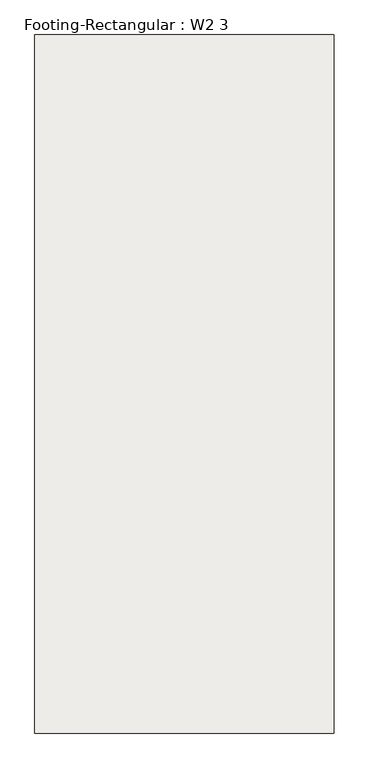
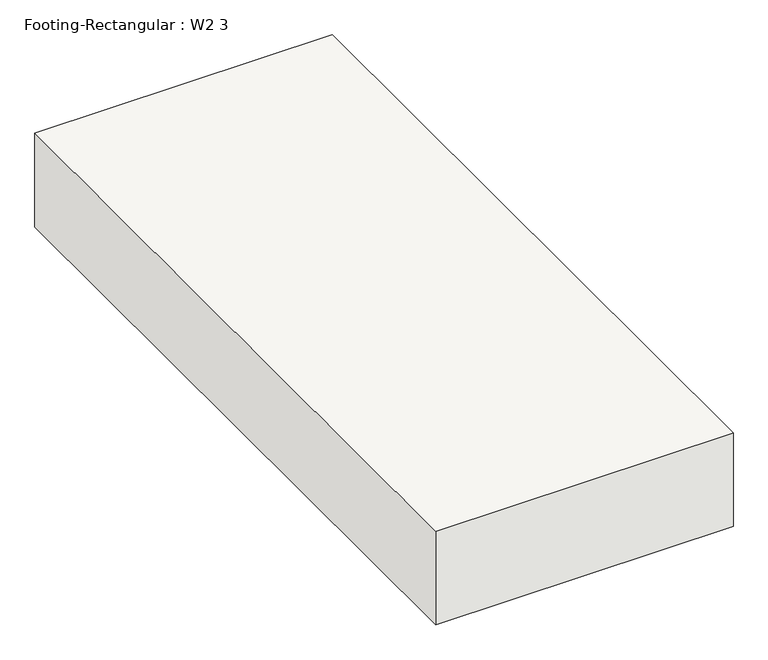
"""IFC4 building model written with IfcOpenShell, lengths in millimetres: slab geometry, Footing-Rectangular : W2 3."""

from ifc_helpers import new_model, si_unit, frame, origin, place, context, project, spatial, polyline, outline, extrude, source, transform, mapped, element, save


def footing_rectangular_w2_3_42326a9c(model_context):
    return source(origin(), model_context, "Body", "SweptSolid", [
        extrude(outline(polyline([(457.2, 1066.8), (457.2, -1066.8), (-457.2, -1066.8), (-457.2, 1066.8), (457.2, 1066.8)])), frame((0.0, 0.0, -304.8), z_axis=(0.0, 0.0, 1.0), x_axis=(1.0, 0.0, 0.0)), (0.0, 0.0, 1.0), 304.8),
    ])


if __name__ == "__main__":
    model = new_model("IFC4")
    model_context = context("Model", 3, world=origin())
    ifc_project = project(units=[si_unit("LENGTHUNIT", "METRE", prefix="MILLI")], contexts=[model_context])
    site = spatial("IfcSite", under=ifc_project)
    building = spatial("IfcBuilding", under=site)
    placement = place(None, origin())
    footing_rectangular_w2_3_shape = footing_rectangular_w2_3_42326a9c(model_context)
    element("IfcSlab", 1, ObjectType="Footing-Rectangular : W2 3", at=placement, inside=building, context=model_context, shape_type="MappedRepresentation", body=[
        mapped(footing_rectangular_w2_3_shape, transform((0.0, 0.0, 0.0), x_axis=(1.0, 0.0, 0.0), y_axis=(0.0, 1.0, 0.0), z_axis=(0.0, 0.0, 1.0))),
    ])
    save(model, "model.ifc")

# Revit data of these elements
# Type "Footing-Rectangular : W2 3"
#   Assembly Code = "A1010100"
#   Width = 3' - 0"
#   Length = 7' - 0"
#   Foundation Thickness = 1' - 0"
#   Structural Material [instance default] = Concrete, Cast-in-Place gray
# Element 1 (IfcSlab, "Footing-Rectangular : W2 3")
#   Materials on its faces: "Concrete, Cast-in-Place gray"
# Materials
#   "Concrete, Cast-in-Place gray": class "Concrete", colour RGB 192 192 192, transparency 0, Description = "Cast-in-place concrete", Cost = 0
